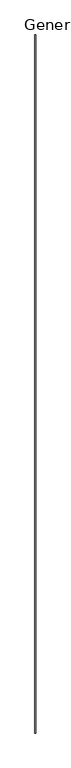
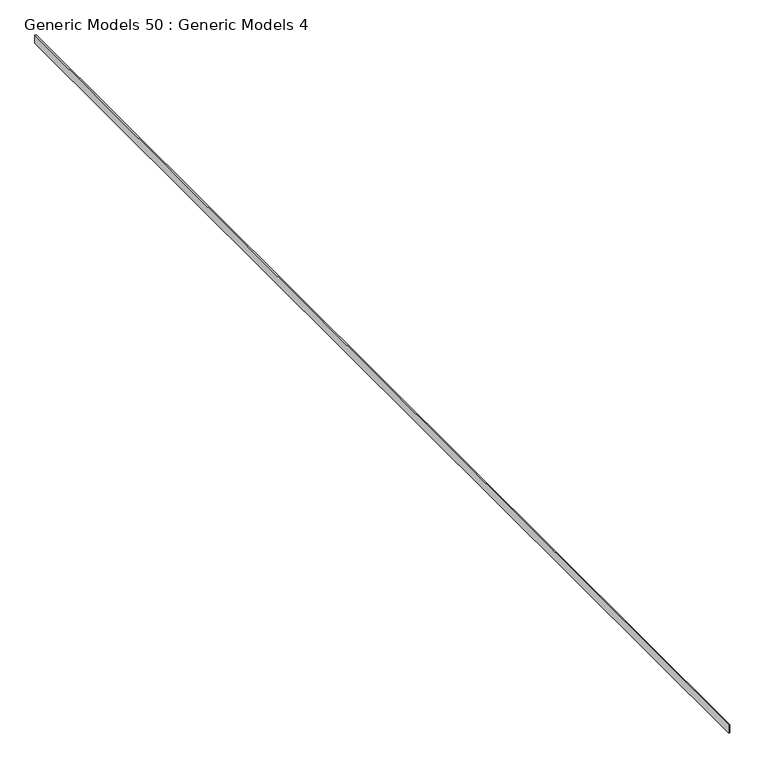
"""IFC4 building model written with IfcOpenShell, lengths in millimetres: proxy geometry, Generic Models 50 : Generic Models 4."""

from ifc_helpers import new_model, si_unit, frame, origin, place, context, project, spatial, polyline, outline, extrude, source, transform, mapped, element, save


def generic_models_50_generic_models_4_0e563b42(model_context):
    return source(origin(), model_context, "Body", "SweptSolid", [
        extrude(outline(polyline([(7253.8514146, -6864.9230338), (7234.8014146, -6864.9230338), (7234.8014146, 11778.6769662), (7253.8514146, 11778.6769662), (7253.8514146, -6864.9230338)])), frame((0.0, 0.0, 126809.341198), z_axis=(0.0, 0.0, 1.0), x_axis=(1.0, 0.0, 0.0)), (0.0, 0.0, 1.0), 132.6610303),
    ])


if __name__ == "__main__":
    model = new_model("IFC4")
    model_context = context("Model", 3, world=origin())
    ifc_project = project(units=[si_unit("LENGTHUNIT", "METRE", prefix="MILLI")], contexts=[model_context])
    site = spatial("IfcSite", under=ifc_project)
    building = spatial("IfcBuilding", under=site)
    placement = place(None, origin())
    generic_models_50_generic_models_4_shape = generic_models_50_generic_models_4_0e563b42(model_context)
    element("IfcBuildingElementProxy", 1, Name="Generic Models 50 : Generic Models 4", ObjectType="Generic Models 50 : Generic Models 4", at=placement, inside=building, context=model_context, shape_type="MappedRepresentation", body=[
        mapped(generic_models_50_generic_models_4_shape, transform((0.0, 0.0, 0.0), x_axis=(1.0, 0.0, 0.0), y_axis=(0.0, 1.0, 0.0), z_axis=(0.0, 0.0, 1.0))),
    ])
    save(model, "model.ifc")

# Revit data of these elements
# Element 1 (IfcBuildingElementProxy, "Generic Models 50 : Generic Models 4")
#   Materials on its faces: "_CDX PLYWOOD - SEE STRUCT DWGs"
# Materials
#   "_CDX PLYWOOD - SEE STRUCT DWGs": class "Generic", colour RGB 98 75 74, transparency 0, Cost = 0
